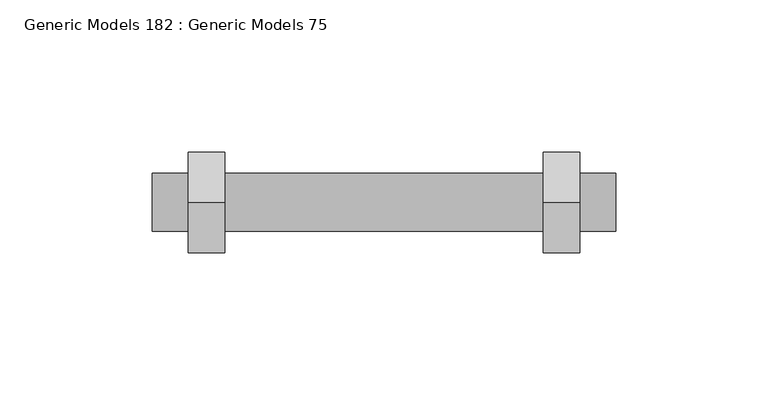
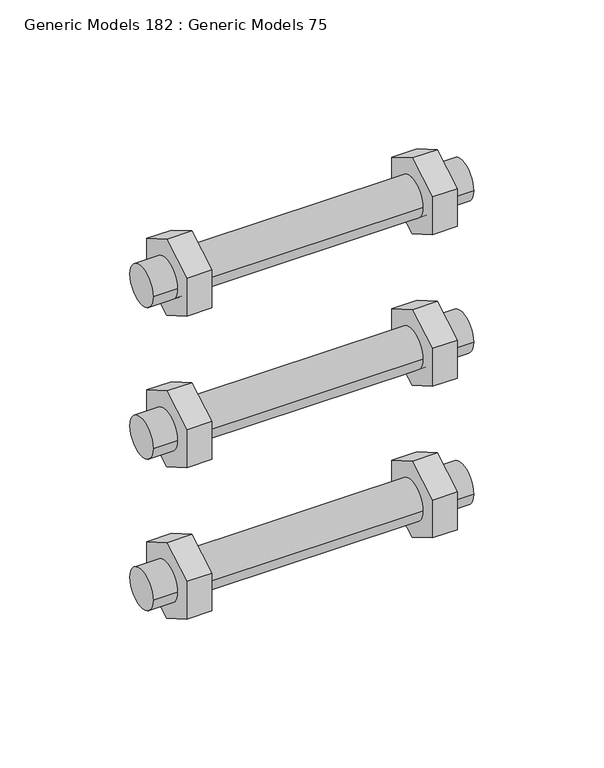
"""IFC4 building model written with IfcOpenShell, lengths in millimetres: proxy geometry, Generic Models 182 : Generic Models 75."""

from ifc_helpers import new_model, si_unit, point, frame, frame_2d, origin, place, context, project, spatial, polyline, circle_curve, trimmed, segment, composite_curve, outline, extrude, source, transform, mapped, element, save


def generic_models_182_generic_models_75_ef481025(model_context):
    return source(origin(), model_context, "Body", "SweptSolid", [
        extrude(outline(polyline([(30636.0571951, 269062.859622), (30636.0571951, 269043.809622), (30619.5594112, 269034.284622), (30603.0616273, 269043.809622), (30603.0616273, 269062.859622), (30619.5594112, 269072.384622), (30636.0571951, 269062.859622)])), frame((31918.2596032, 0.0, 0.0), z_axis=(1.0, 0.0, 0.0), x_axis=(0.0, 1.0, 0.0)), (0.0, 0.0, 1.0), 11.90625),
        extrude(outline(polyline([(30636.0571951, 268986.659622), (30636.0571951, 268967.609622), (30619.5594112, 268958.084622), (30603.0616273, 268967.609622), (30603.0616273, 268986.659622), (30619.5594112, 268996.184622), (30636.0571951, 268986.659622)])), frame((31918.2596032, 0.0, 0.0), z_axis=(1.0, 0.0, 0.0), x_axis=(0.0, 1.0, 0.0)), (0.0, 0.0, 1.0), 11.90625),
        extrude(outline(polyline([(30636.0571951, 268910.459622), (30636.0571951, 268891.409622), (30619.5594112, 268881.884622), (30603.0616273, 268891.409622), (30603.0616273, 268910.459622), (30619.5594112, 268919.984622), (30636.0571951, 268910.459622)])), frame((31918.2596032, 0.0, 0.0), z_axis=(1.0, 0.0, 0.0), x_axis=(0.0, 1.0, 0.0)), (0.0, 0.0, 1.0), 11.90625),
        extrude(outline(polyline([(30636.0571951, 269062.859622), (30636.0571951, 269043.809622), (30619.5594112, 269034.284622), (30603.0616273, 269043.809622), (30603.0616273, 269062.859622), (30619.5594112, 269072.384622), (30636.0571951, 269062.859622)])), frame((31801.5783532, 0.0, 0.0), z_axis=(1.0, 0.0, 0.0), x_axis=(0.0, 1.0, 0.0)), (0.0, 0.0, 1.0), 11.90625),
        extrude(outline(polyline([(30636.0571951, 268986.659622), (30636.0571951, 268967.609622), (30619.5594112, 268958.084622), (30603.0616273, 268967.609622), (30603.0616273, 268986.659622), (30619.5594112, 268996.184622), (30636.0571951, 268986.659622)])), frame((31801.5783532, 0.0, 0.0), z_axis=(1.0, 0.0, 0.0), x_axis=(0.0, 1.0, 0.0)), (0.0, 0.0, 1.0), 11.90625),
        extrude(outline(polyline([(30636.0571951, 268910.459622), (30636.0571951, 268891.409622), (30619.5594112, 268881.884622), (30603.0616273, 268891.409622), (30603.0616273, 268910.459622), (30619.5594112, 268919.984622), (30636.0571951, 268910.459622)])), frame((31801.5783532, 0.0, 0.0), z_axis=(1.0, 0.0, 0.0), x_axis=(0.0, 1.0, 0.0)), (0.0, 0.0, 1.0), 11.90625),
        extrude(outline(composite_curve([segment(trimmed(circle_curve(frame_2d((30619.5594112, 268977.134622)), 9.525), [point((30610.0344112, 268977.134622))], [point((30629.0844112, 268977.134622))], False, "CARTESIAN"), True, "CONTINUOUS"), segment(trimmed(circle_curve(frame_2d((30619.5594112, 268977.134622)), 9.525), [point((30629.0844112, 268977.134622))], [point((30610.0344112, 268977.134622))], False, "CARTESIAN"), True, "CONTINUOUS")], self_intersect=False)), frame((31789.6721032, 0.0, 0.0), z_axis=(1.0, 0.0, 0.0), x_axis=(0.0, 1.0, 0.0)), (0.0, 0.0, 1.0), 152.4),
        extrude(outline(composite_curve([segment(trimmed(circle_curve(frame_2d((30619.5594112, 268900.934622)), 9.525), [point((30610.0344112, 268900.934622))], [point((30629.0844112, 268900.934622))], False, "CARTESIAN"), True, "CONTINUOUS"), segment(trimmed(circle_curve(frame_2d((30619.5594112, 268900.934622)), 9.525), [point((30629.0844112, 268900.934622))], [point((30610.0344112, 268900.934622))], False, "CARTESIAN"), True, "CONTINUOUS")], self_intersect=False)), frame((31789.6721032, 0.0, 0.0), z_axis=(1.0, 0.0, 0.0), x_axis=(0.0, 1.0, 0.0)), (0.0, 0.0, 1.0), 152.4),
        extrude(outline(composite_curve([segment(trimmed(circle_curve(frame_2d((30619.5594112, 269053.334622)), 9.525), [point((30610.0344112, 269053.334622))], [point((30629.0844112, 269053.334622))], False, "CARTESIAN"), True, "CONTINUOUS"), segment(trimmed(circle_curve(frame_2d((30619.5594112, 269053.334622)), 9.525), [point((30629.0844112, 269053.334622))], [point((30610.0344112, 269053.334622))], False, "CARTESIAN"), True, "CONTINUOUS")], self_intersect=False)), frame((31789.6721032, 0.0, 0.0), z_axis=(1.0, 0.0, 0.0), x_axis=(0.0, 1.0, 0.0)), (0.0, 0.0, 1.0), 152.4),
    ])


if __name__ == "__main__":
    model = new_model("IFC4")
    model_context = context("Model", 3, world=origin())
    ifc_project = project(units=[si_unit("LENGTHUNIT", "METRE", prefix="MILLI")], contexts=[model_context])
    site = spatial("IfcSite", under=ifc_project)
    building = spatial("IfcBuilding", under=site)
    placement = place(None, origin())
    generic_models_182_generic_models_75_shape = generic_models_182_generic_models_75_ef481025(model_context)
    element("IfcBuildingElementProxy", 1, Name="Generic Models 182 : Generic Models 75", ObjectType="Generic Models 182 : Generic Models 75", at=placement, inside=building, context=model_context, shape_type="MappedRepresentation", body=[
        mapped(generic_models_182_generic_models_75_shape, transform((0.0, 0.0, 0.0), x_axis=(1.0, 0.0, 0.0), y_axis=(0.0, 1.0, 0.0), z_axis=(0.0, 0.0, 1.0))),
    ])
    save(model, "model.ifc")
